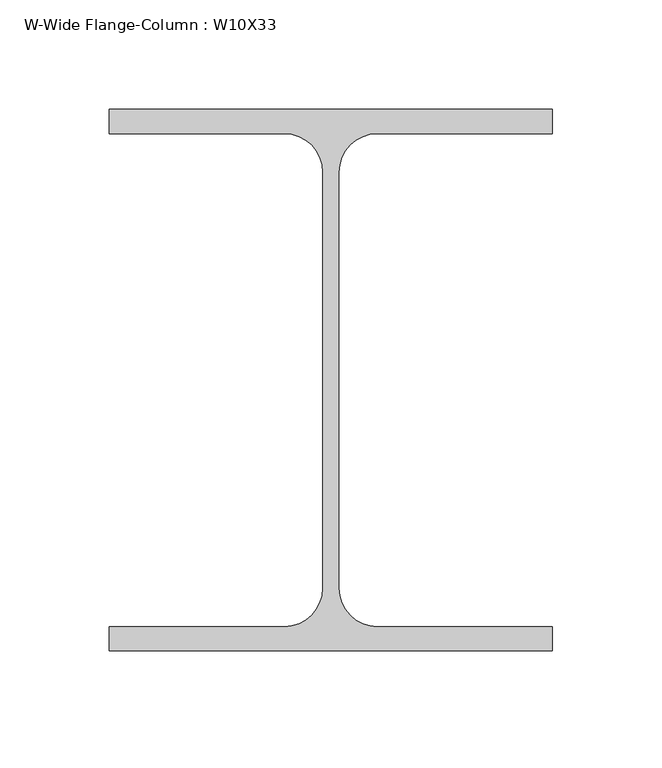
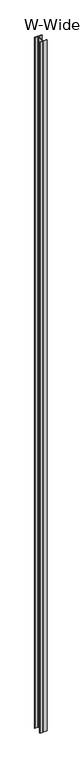
"""IFC4 building model written with IfcOpenShell, lengths in millimetres: column geometry, W-Wide Flange-Column : W10X33."""

import ifcopenshell
import ifcopenshell.guid

model = None  # the IFC model being written
_history = None  # IfcOwnerHistory: only IFC2X3 demands one
_inside = {}  # id of a spatial element -> (the spatial element, [elements in it])
_under = {}  # id of a project, library or spatial element -> (it, [spatial elements below it])
_declared = {}  # id of a project -> (the project, [libraries it declares])
_typed = {}  # id of a type object -> (the type object, [elements of that type])
_made_of = {}  # id of a material, layer set ... -> (it, [elements and type objects made of it])


def new_model(schema):
    """Start an empty IFC model of exactly this schema.

    Asked for "IFC4X3", IfcOpenShell would pick the latest addendum, in which some entities
    have other attributes; the version numbers below select the first issue.
    IFC2X3 requires an IfcOwnerHistory on every rooted entity: one is made here for all.
    """
    global model, _history
    if schema == "IFC4X3":
        model = ifcopenshell.file(schema_version=(4, 3, 0, 0))
    else:
        model = ifcopenshell.file(schema=schema)
    _inside.clear()
    _under.clear()
    _declared.clear()
    _typed.clear()
    _made_of.clear()
    _history = None
    if model.schema == "IFC2X3":
        org = make("IfcOrganization", Name="unknown")
        user = make(
            "IfcPersonAndOrganization",
            ThePerson=make("IfcPerson", FamilyName="unknown"),
            TheOrganization=org,
        )
        app = make(
            "IfcApplication",
            ApplicationDeveloper=org,
            Version="unknown",
            ApplicationFullName="unknown",
            ApplicationIdentifier="unknown",
        )
        _history = make(
            "IfcOwnerHistory",
            OwningUser=user,
            OwningApplication=app,
            ChangeAction="ADDED",
            CreationDate=0,
        )
    return model


def make(cls, **values):
    """One entity of the class cls with the attributes given. An attribute that is None is left unset."""
    return model.create_entity(
        cls, **{name: value for name, value in values.items() if value is not None}
    )


def rooted(cls, **values):
    """An entity with a GlobalId (a new one), such as an element, a storey or a relation."""
    return make(cls, GlobalId=ifcopenshell.guid.new(), OwnerHistory=_history, **values)


def si_unit(unit_type, name, prefix=None):
    """IfcSIUnit, for example si_unit("LENGTHUNIT", "METRE", prefix="MILLI")."""
    return make("IfcSIUnit", UnitType=unit_type, Prefix=prefix, Name=name)


def assignment(units):
    """IfcUnitAssignment: the units of a project."""
    return None if units is None else make("IfcUnitAssignment", Units=units)


def point(xyz):
    """IfcCartesianPoint."""
    return None if xyz is None else make("IfcCartesianPoint", Coordinates=xyz)


def direction(xyz):
    """IfcDirection."""
    return None if xyz is None else make("IfcDirection", DirectionRatios=xyz)


def frame(location, z_axis=None, x_axis=None):
    """IfcAxis2Placement3D, a coordinate frame: its origin and axes. An axis left out is left unset."""
    return make(
        "IfcAxis2Placement3D",
        Location=point(location),
        Axis=direction(z_axis),
        RefDirection=direction(x_axis),
    )


def frame_2d(location, x_axis=None):
    """IfcAxis2Placement2D, a coordinate frame in the plane: its origin and x axis."""
    return make(
        "IfcAxis2Placement2D", Location=point(location), RefDirection=direction(x_axis)
    )


def origin():
    """The frame at (0, 0, 0) with its axes left unset."""
    return frame((0.0, 0.0, 0.0))


def place(relative_to, where):
    """IfcLocalPlacement: puts the frame where relative to a parent placement (None: the world)."""
    return make(
        "IfcLocalPlacement", PlacementRelTo=relative_to, RelativePlacement=where
    )


def context(
    kind, dimensions, precision=None, world=None, true_north=None, identifier=None
):
    """IfcGeometricRepresentationContext, for example the 3D "Model" context."""
    return make(
        "IfcGeometricRepresentationContext",
        ContextIdentifier=identifier,
        ContextType=kind,
        CoordinateSpaceDimension=dimensions,
        Precision=precision,
        WorldCoordinateSystem=world,
        TrueNorth=true_north,
    )


def project(units=None, contexts=None):
    """IfcProject with its units and contexts."""
    return rooted(
        "IfcProject",
        Name="project",
        RepresentationContexts=contexts,
        UnitsInContext=assignment(units),
    )


def spatial(cls, under=None, at=None, **own):
    """A site, building, storey or space (cls), placed at a placement, below another one or the project."""
    s = rooted(cls, ObjectPlacement=at, **own)
    if under is not None:
        _under.setdefault(under.id(), (under, []))[1].append(s)
    return s


def polyline(points):
    """IfcPolyline through the points."""
    return make("IfcPolyline", Points=[point(p) for p in points])


def circle_curve(where, radius):
    """IfcCircle in the frame where."""
    return make("IfcCircle", Position=where, Radius=radius)


def trimmed(basis, trim1, trim2, sense, master):
    """IfcTrimmedCurve: the piece of a basis curve between two trims."""
    return make(
        "IfcTrimmedCurve",
        BasisCurve=basis,
        Trim1=trim1,
        Trim2=trim2,
        SenseAgreement=sense,
        MasterRepresentation=master,
    )


def segment(curve, same_sense, transition):
    """IfcCompositeCurveSegment."""
    return make(
        "IfcCompositeCurveSegment",
        Transition=transition,
        SameSense=same_sense,
        ParentCurve=curve,
    )


def composite_curve(segments, self_intersect=None):
    """IfcCompositeCurve: segments joined end to end."""
    return make("IfcCompositeCurve", Segments=segments, SelfIntersect=self_intersect)


def outline(outer, holes=None, kind="AREA"):
    """IfcArbitraryClosedProfileDef: a profile drawn as a closed curve; with holes, ...WithVoids."""
    if holes is None:
        return make("IfcArbitraryClosedProfileDef", ProfileType=kind, OuterCurve=outer)
    return make(
        "IfcArbitraryProfileDefWithVoids",
        ProfileType=kind,
        OuterCurve=outer,
        InnerCurves=holes,
    )


def extrude(swept, where, along, depth):
    """IfcExtrudedAreaSolid: the profile swept, set in the frame where, extruded along a direction by depth."""
    return make(
        "IfcExtrudedAreaSolid",
        SweptArea=swept,
        Position=where,
        ExtrudedDirection=direction(along),
        Depth=depth,
    )


def shape(context_of_items, identifier, shape_type, items):
    """IfcShapeRepresentation: the items that make up one representation, for example the "Body"."""
    return make(
        "IfcShapeRepresentation",
        ContextOfItems=context_of_items,
        RepresentationIdentifier=identifier,
        RepresentationType=shape_type,
        Items=items,
    )


def source(mapping_origin, context_of_items, identifier, shape_type, items):
    """IfcRepresentationMap: a shape defined once, which mapped items show again and again."""
    return make(
        "IfcRepresentationMap",
        MappingOrigin=mapping_origin,
        MappedRepresentation=shape(context_of_items, identifier, shape_type, items),
    )


def transform(
    local_origin,
    x_axis=None,
    y_axis=None,
    z_axis=None,
    scale=None,
    scale2=None,
    scale3=None,
    uniform=True,
):
    """IfcCartesianTransformationOperator3D, or its non-uniform kind. x_axis, y_axis, z_axis: its Axis1, 2, 3."""
    if uniform:
        return make(
            "IfcCartesianTransformationOperator3D",
            Axis1=direction(x_axis),
            Axis2=direction(y_axis),
            LocalOrigin=point(local_origin),
            Scale=scale,
            Axis3=direction(z_axis),
        )
    return make(
        "IfcCartesianTransformationOperator3DnonUniform",
        Axis1=direction(x_axis),
        Axis2=direction(y_axis),
        LocalOrigin=point(local_origin),
        Scale=scale,
        Axis3=direction(z_axis),
        Scale2=scale2,
        Scale3=scale3,
    )


def mapped(mapping_source, mapping_target):
    """IfcMappedItem: shows the shape of a source again, moved by a transform."""
    return make(
        "IfcMappedItem", MappingSource=mapping_source, MappingTarget=mapping_target
    )


def made_of(thing, what):
    """Note that an element or type object is made of a material, layer set ...; save() writes the relation."""
    if what is not None:
        _made_of.setdefault(what.id(), (what, []))[1].append(thing)
    return thing


def element(
    cls,
    number,
    at=None,
    inside=None,
    cuts=None,
    type_object=None,
    material=None,
    context=None,
    identifier="Body",
    shape_type=None,
    held_by="IfcProductDefinitionShape",
    body=None,
    shapes=None,
    **own,
):
    """One element of the class cls, such as IfcWall. Its Tag is "e" and its number.

    at: its placement. inside: the storey or other place that contains it. cuts: it is an
    opening in that element (IfcRelVoidsElement). A single representation is given by context,
    identifier, shape_type and body (its items); several are given by shapes. held_by: the class
    of the entity that holds the representations. save() writes the other relations.
    """
    e = rooted(cls, Tag="e%d" % number, ObjectPlacement=at, **own)
    if body is not None:
        shapes = [shape(context, identifier, shape_type, body)]
    if shapes is not None:
        e.Representation = make(held_by, Representations=shapes)
    if inside is not None:
        _inside.setdefault(inside.id(), (inside, []))[1].append(e)
    if cuts is not None:
        rooted(
            "IfcRelVoidsElement", RelatingBuildingElement=cuts, RelatedOpeningElement=e
        )
    if type_object is not None:
        _typed.setdefault(type_object.id(), (type_object, []))[1].append(e)
    return made_of(e, material)


def aggregate(whole, parts):
    """IfcRelAggregates: a whole, such as a stair, and the parts it consists of."""
    return rooted("IfcRelAggregates", RelatingObject=whole, RelatedObjects=parts)


def save(model, path):
    """Write the relations noted so far, then the file.

    IfcRelAggregates (storeys below a building ...), IfcRelContainedInSpatialStructure (elements
    in a storey), IfcRelDefinesByType, IfcRelAssociatesMaterial and IfcRelDeclares: one each for
    every whole, place, type object, material and project.
    """
    for whole, parts in _under.values():
        aggregate(whole, parts)
    for where, things in _inside.values():
        rooted(
            "IfcRelContainedInSpatialStructure",
            RelatedElements=things,
            RelatingStructure=where,
        )
    for kind, things in _typed.values():
        rooted("IfcRelDefinesByType", RelatedObjects=things, RelatingType=kind)
    for what, things in _made_of.values():
        rooted("IfcRelAssociatesMaterial", RelatedObjects=things, RelatingMaterial=what)
    for by, libraries in _declared.values():
        rooted("IfcRelDeclares", RelatingContext=by, RelatedDefinitions=libraries)
    model.write(path)


def w_wide_flange_column_w10x33_7ea207c2(model_context):
    return source(origin(), model_context, "Body", "SweptSolid", [
        extrude(outline(composite_curve([segment(polyline([(101.092, 123.571), (101.092, 112.522), (21.209, 112.522)]), True, "CONTINUOUS"), segment(trimmed(circle_curve(frame_2d((21.209, 94.996)), 17.526), [point((21.209, 112.522))], [point((3.683, 94.996))], True, "CARTESIAN"), True, "CONTINUOUS"), segment(polyline([(3.683, 94.996), (3.683, -94.996)]), True, "CONTINUOUS"), segment(trimmed(circle_curve(frame_2d((21.209, -94.996)), 17.526), [point((3.683, -94.996))], [point((21.209, -112.522))], True, "CARTESIAN"), True, "CONTINUOUS"), segment(polyline([(21.209, -112.522), (101.092, -112.522), (101.092, -123.571), (-101.092, -123.571), (-101.092, -112.522), (-21.209, -112.522)]), True, "CONTINUOUS"), segment(trimmed(circle_curve(frame_2d((-21.209, -94.996)), 17.526), [point((-21.209, -112.522))], [point((-3.683, -94.996))], True, "CARTESIAN"), True, "CONTINUOUS"), segment(polyline([(-3.683, -94.996), (-3.683, 94.996)]), True, "CONTINUOUS"), segment(trimmed(circle_curve(frame_2d((-21.209, 94.996)), 17.526), [point((-3.683, 94.996))], [point((-21.209, 112.522))], True, "CARTESIAN"), True, "CONTINUOUS"), segment(polyline([(-21.209, 112.522), (-101.092, 112.522), (-101.092, 123.571), (101.092, 123.571)]), True, "CONTINUOUS")], self_intersect=False)), frame((0.0, 0.0, 9163.05), z_axis=(0.0, 0.0, 1.0), x_axis=(1.0, 0.0, 0.0)), (0.0, 0.0, 1.0), 20402.55),
    ])


if __name__ == "__main__":
    model = new_model("IFC4")
    model_context = context("Model", 3, world=origin())
    ifc_project = project(units=[si_unit("LENGTHUNIT", "METRE", prefix="MILLI")], contexts=[model_context])
    site = spatial("IfcSite", under=ifc_project)
    building = spatial("IfcBuilding", under=site)
    placement = place(None, origin())
    w_wide_flange_column_w10x33_shape = w_wide_flange_column_w10x33_7ea207c2(model_context)
    element("IfcColumn", 1, ObjectType="W-Wide Flange-Column : W10X33", at=placement, inside=building, context=model_context, shape_type="MappedRepresentation", body=[
        mapped(w_wide_flange_column_w10x33_shape, transform((0.0, 0.0, 0.0), x_axis=(1.0, 0.0, 0.0), y_axis=(0.0, 1.0, 0.0), z_axis=(0.0, 0.0, 1.0))),
    ])
    save(model, "model.ifc")

# Revit data of these elements
# Type "W-Wide Flange-Column : W10X33"
#   Assembly Code = "B10"
#   W = 33
#   bf = 0' - 7.96"
#   d = 0' - 9.73"
#   k = 0' - 1 1/8"
#   kr = 0' - 0.69"
#   tf = 0' - 0.435"
#   tw = 0' - 0.29"
#   A = 0.0674306 SF
#   Structural Material [instance default] = Steel ASTM A992
# Element 1 (IfcColumn, "W-Wide Flange-Column : W10X33")
#   Materials on its faces: "Steel ASTM A992"
# Materials
#   "Steel ASTM A992": class "Metal", colour RGB 199 199 199, transparency 0, Description = "Structural steel 50ksi", Cost = 0
